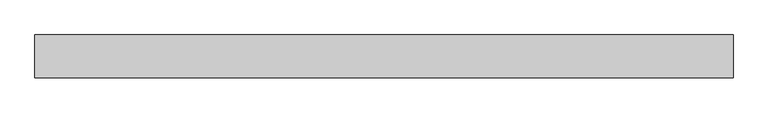
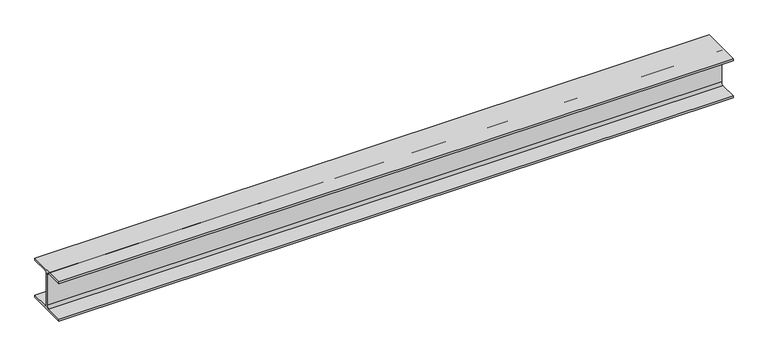
"""IFC4 building model written with IfcOpenShell, lengths in millimetres: beam geometry, 0912_Steel Framing_H-KSD3502 : H_SB_ASB_H-300x300x10x15."""

from ifc_helpers import new_model, si_unit, point, frame, frame_2d, origin, place, context, project, spatial, polyline, circle_curve, trimmed, segment, composite_curve, outline, extrude, source, transform, mapped, element, save


def beam_ed173aaa(model_context):
    return source(origin(), model_context, "Body", "SweptSolid", [
        extrude(outline(composite_curve([segment(polyline([(-150.0, -135.0), (-23.0, -135.0)]), True, "CONTINUOUS"), segment(trimmed(circle_curve(frame_2d((-23.0, -117.0)), 18.0), [point((-23.0, -135.0))], [point((-5.0, -117.0))], True, "CARTESIAN"), True, "CONTINUOUS"), segment(polyline([(-5.0, -117.0), (-5.0, 117.0)]), True, "CONTINUOUS"), segment(trimmed(circle_curve(frame_2d((-23.0, 117.0)), 18.0), [point((-5.0, 117.0))], [point((-23.0, 135.0))], True, "CARTESIAN"), True, "CONTINUOUS"), segment(polyline([(-23.0, 135.0), (-150.0, 135.0), (-150.0, 150.0), (150.0, 150.0), (150.0, 135.0), (23.0, 135.0)]), True, "CONTINUOUS"), segment(trimmed(circle_curve(frame_2d((23.0, 117.0)), 18.0), [point((23.0, 135.0))], [point((5.0, 117.0))], True, "CARTESIAN"), True, "CONTINUOUS"), segment(polyline([(5.0, 117.0), (5.0, -117.0)]), True, "CONTINUOUS"), segment(trimmed(circle_curve(frame_2d((23.0, -117.0)), 18.0), [point((5.0, -117.0))], [point((23.0, -135.0))], True, "CARTESIAN"), True, "CONTINUOUS"), segment(polyline([(23.0, -135.0), (150.0, -135.0), (150.0, -150.0), (-150.0, -150.0), (-150.0, -135.0)]), True, "CONTINUOUS")], self_intersect=False)), frame((-2479.7628546, 0.0, 0.0), z_axis=(1.0, 0.0, 0.0), x_axis=(0.0, 1.0, 0.0)), (0.0, 0.0, 1.0), 4891.0868037),
    ])


if __name__ == "__main__":
    model = new_model("IFC4")
    model_context = context("Model", 3, world=origin())
    ifc_project = project(units=[si_unit("LENGTHUNIT", "METRE", prefix="MILLI")], contexts=[model_context])
    site = spatial("IfcSite", under=ifc_project)
    building = spatial("IfcBuilding", under=site)
    placement = place(None, origin())
    beam_shape = beam_ed173aaa(model_context)
    element("IfcBeam", 1, ObjectType="0912_Steel Framing_H-KSD3502 : H_SB_ASB_H-300x300x10x15", at=placement, inside=building, context=model_context, shape_type="MappedRepresentation", body=[
        mapped(beam_shape, transform((0.0, 0.0, 0.0), x_axis=(1.0, 0.0, 0.0), y_axis=(0.0, 1.0, 0.0), z_axis=(0.0, 0.0, 1.0))),
    ])
    save(model, "model.ifc")

# Revit data of these elements
# Type "0912_Steel Framing_H-KSD3502 : H_SB_ASB_H-300x300x10x15"
#   H_WM Code_1 = "S01AA001-00001 | Main Steel Structure Fabrication Work | Shelter/Building | Heavy Steel - Standard (Weight≥90KG/M) | Material: (   )"
#   H_WM Code_2 = "S03AA027-00001 | Main Steel Structure Erection Work | Shelter/Building | Heavy Steel (Weight≥90KG/M) | Material: (   )"
#   H_WM Code_3 = "S01AA010-00001 | Main Steel Structure Fabrication Work | Shelter/Building | Steel Painting/Coating | for Non-Fireproofed Steel Surface, Surface Preparation, Primer, Second & Final Coat | Material: (   )"
#   H_Q'ty Cal Type Tag = "SB-Q2"
#   Width = 30.0 cm
#   Web Thickness = 1.0 cm
#   Web Fillet = 1.8 cm
#   Warping Constant = 1370000.0 cm⁶
#   W = 0
#   Torsional Moment of Inertia = 77.00 cm⁴
#   Section Area = 119.8 cm²
#   Plastic Modulus weak axis = 684.0 cm³
#   Plastic Modulus strong axis = 1500.0 cm³
#   Perimeter = 1.75 m²/m
#   Nominal Weight = 94.00 kgf/m
#   Moment of Inertia weak axis = 6750.00 cm⁴
#   Moment of Inertia strong axis = 20400.00 cm⁴
#   Height = 30.0 cm
#   Flange Thickness = 1.5 cm
#   Elastic Modulus weak axis = 450.0 cm³
#   Elastic Modulus strong axis = 1360.0 cm³
#   Centroid Vertical = 15.0 cm
#   Centroid Horizontal = 15.0 cm
#   Ix = 204000000
#   Length [instance default] = 1.5240 m
#   Zx = 1500000
#   b = 0.3000 m
#   h = 0.3000 m
#   r = 0.0180 m
#   s = 0.0100 m
#   t = 0.0150 m
#   A = 0.01198 m²
#   Structural Material [instance default] = Steel, 45-345
#   Assembly Code = ""
# Element 1 (IfcBeam, "0912_Steel Framing_H-KSD3502 : H_SB_ASB_H-300x300x10x15")
#   Structural Material = none
# Materials
#   "Steel, 45-345": class "Metal", colour RGB 189 187 185, transparency 0, Description = "Steel 345 MPa", Cost = 0
